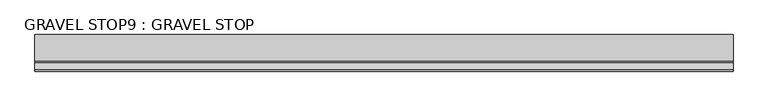
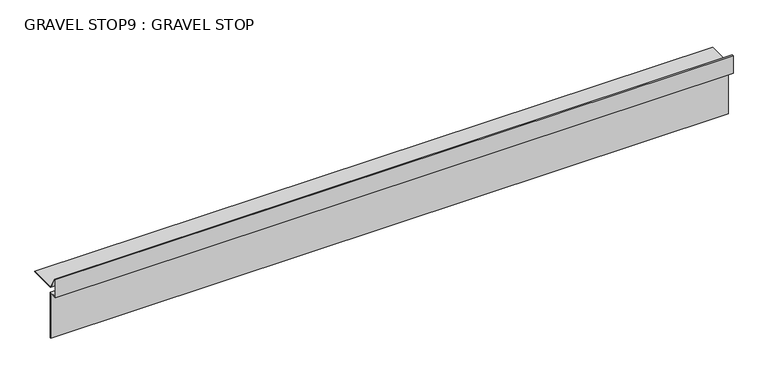
"""IFC4 building model written with IfcOpenShell, lengths in millimetres: proxy geometry, GRAVEL STOP9 : GRAVEL STOP."""

from ifc_helpers import new_model, si_unit, frame, origin, place, context, project, spatial, polyline, outline, extrude, source, transform, mapped, element, save


def gravel_stop9_gravel_stop_f17445ac(model_context):
    return source(origin(), model_context, "Body", "SweptSolid", [
        extrude(outline(polyline([(-5580.0356381, 40278.1940248), (-5577.0037237, 40279.0064238), (-5556.3332702, 40243.204148), (-5552.58096, 40241.0377507), (-5475.1230533, 40241.0377507), (-5475.1230533, 40239.6266397), (-5552.959066, 40239.6266397), (-5557.3662751, 40242.1711431), (-5577.6843899, 40277.3631503), (-5578.6245271, 40277.1112413), (-5578.6245271, 40224.6266397), (-5554.2847895, 40224.6266397), (-5554.2847895, 40081.6491197), (-5555.6959005, 40081.6491197), (-5555.6959005, 40223.2155287), (-5580.0356381, 40223.2155287), (-5580.0356381, 40278.1940248)])), frame((12382.7678845, 0.0, 0.0), z_axis=(1.0, 0.0, 0.0), x_axis=(0.0, 1.0, 0.0)), (0.0, 0.0, 1.0), 2000.25),
    ])


if __name__ == "__main__":
    model = new_model("IFC4")
    model_context = context("Model", 3, world=origin())
    ifc_project = project(units=[si_unit("LENGTHUNIT", "METRE", prefix="MILLI")], contexts=[model_context])
    site = spatial("IfcSite", under=ifc_project)
    building = spatial("IfcBuilding", under=site)
    placement = place(None, origin())
    gravel_stop9_gravel_stop_shape = gravel_stop9_gravel_stop_f17445ac(model_context)
    element("IfcBuildingElementProxy", 1, Name="GRAVEL STOP9 : GRAVEL STOP", ObjectType="GRAVEL STOP9 : GRAVEL STOP", at=placement, inside=building, context=model_context, shape_type="MappedRepresentation", body=[
        mapped(gravel_stop9_gravel_stop_shape, transform((0.0, 0.0, 0.0), x_axis=(1.0, 0.0, 0.0), y_axis=(0.0, 1.0, 0.0), z_axis=(0.0, 0.0, 1.0))),
    ])
    save(model, "model.ifc")

# Revit data of these elements
# Type "GRAVEL STOP9 : GRAVEL STOP"
#   NameOverride = "GRAVEL STOP"
# Element 1 (IfcBuildingElementProxy, "GRAVEL STOP9 : GRAVEL STOP")
#   Materials on its faces: "GRAVEL STOP REQUIRED WITH GRAVEL SURFACE SYSTEMS"
# Materials
#   "GRAVEL STOP REQUIRED WITH GRAVEL SURFACE SYSTEMS": class "Unassigned", colour RGB 170 170 127, transparency 0, Cost = 0
